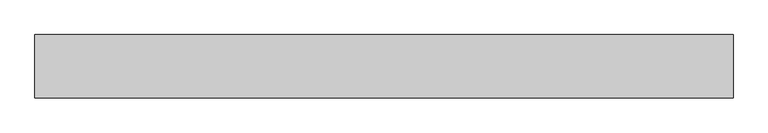
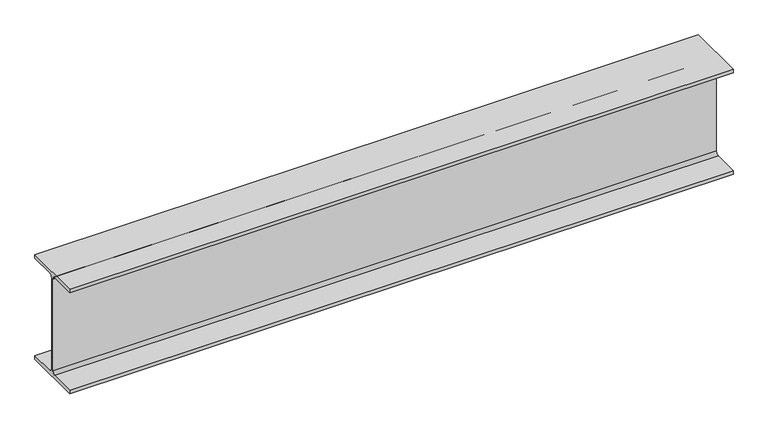
"""IFC4 building model written with IfcOpenShell, lengths in millimetres: beam geometry, Old_Steel Beam_H-KSD3502 : H_SB_ASB_H-200×200x8x12."""

import ifcopenshell
import ifcopenshell.guid

model = None  # the IFC model being written
_history = None  # IfcOwnerHistory: only IFC2X3 demands one
_inside = {}  # id of a spatial element -> (the spatial element, [elements in it])
_under = {}  # id of a project, library or spatial element -> (it, [spatial elements below it])
_declared = {}  # id of a project -> (the project, [libraries it declares])
_typed = {}  # id of a type object -> (the type object, [elements of that type])
_made_of = {}  # id of a material, layer set ... -> (it, [elements and type objects made of it])


def new_model(schema):
    """Start an empty IFC model of exactly this schema.

    Asked for "IFC4X3", IfcOpenShell would pick the latest addendum, in which some entities
    have other attributes; the version numbers below select the first issue.
    IFC2X3 requires an IfcOwnerHistory on every rooted entity: one is made here for all.
    """
    global model, _history
    if schema == "IFC4X3":
        model = ifcopenshell.file(schema_version=(4, 3, 0, 0))
    else:
        model = ifcopenshell.file(schema=schema)
    _inside.clear()
    _under.clear()
    _declared.clear()
    _typed.clear()
    _made_of.clear()
    _history = None
    if model.schema == "IFC2X3":
        org = make("IfcOrganization", Name="unknown")
        user = make(
            "IfcPersonAndOrganization",
            ThePerson=make("IfcPerson", FamilyName="unknown"),
            TheOrganization=org,
        )
        app = make(
            "IfcApplication",
            ApplicationDeveloper=org,
            Version="unknown",
            ApplicationFullName="unknown",
            ApplicationIdentifier="unknown",
        )
        _history = make(
            "IfcOwnerHistory",
            OwningUser=user,
            OwningApplication=app,
            ChangeAction="ADDED",
            CreationDate=0,
        )
    return model


def make(cls, **values):
    """One entity of the class cls with the attributes given. An attribute that is None is left unset."""
    return model.create_entity(
        cls, **{name: value for name, value in values.items() if value is not None}
    )


def rooted(cls, **values):
    """An entity with a GlobalId (a new one), such as an element, a storey or a relation."""
    return make(cls, GlobalId=ifcopenshell.guid.new(), OwnerHistory=_history, **values)


def si_unit(unit_type, name, prefix=None):
    """IfcSIUnit, for example si_unit("LENGTHUNIT", "METRE", prefix="MILLI")."""
    return make("IfcSIUnit", UnitType=unit_type, Prefix=prefix, Name=name)


def assignment(units):
    """IfcUnitAssignment: the units of a project."""
    return None if units is None else make("IfcUnitAssignment", Units=units)


def point(xyz):
    """IfcCartesianPoint."""
    return None if xyz is None else make("IfcCartesianPoint", Coordinates=xyz)


def direction(xyz):
    """IfcDirection."""
    return None if xyz is None else make("IfcDirection", DirectionRatios=xyz)


def frame(location, z_axis=None, x_axis=None):
    """IfcAxis2Placement3D, a coordinate frame: its origin and axes. An axis left out is left unset."""
    return make(
        "IfcAxis2Placement3D",
        Location=point(location),
        Axis=direction(z_axis),
        RefDirection=direction(x_axis),
    )


def frame_2d(location, x_axis=None):
    """IfcAxis2Placement2D, a coordinate frame in the plane: its origin and x axis."""
    return make(
        "IfcAxis2Placement2D", Location=point(location), RefDirection=direction(x_axis)
    )


def origin():
    """The frame at (0, 0, 0) with its axes left unset."""
    return frame((0.0, 0.0, 0.0))


def place(relative_to, where):
    """IfcLocalPlacement: puts the frame where relative to a parent placement (None: the world)."""
    return make(
        "IfcLocalPlacement", PlacementRelTo=relative_to, RelativePlacement=where
    )


def context(
    kind, dimensions, precision=None, world=None, true_north=None, identifier=None
):
    """IfcGeometricRepresentationContext, for example the 3D "Model" context."""
    return make(
        "IfcGeometricRepresentationContext",
        ContextIdentifier=identifier,
        ContextType=kind,
        CoordinateSpaceDimension=dimensions,
        Precision=precision,
        WorldCoordinateSystem=world,
        TrueNorth=true_north,
    )


def project(units=None, contexts=None):
    """IfcProject with its units and contexts."""
    return rooted(
        "IfcProject",
        Name="project",
        RepresentationContexts=contexts,
        UnitsInContext=assignment(units),
    )


def spatial(cls, under=None, at=None, **own):
    """A site, building, storey or space (cls), placed at a placement, below another one or the project."""
    s = rooted(cls, ObjectPlacement=at, **own)
    if under is not None:
        _under.setdefault(under.id(), (under, []))[1].append(s)
    return s


def polyline(points):
    """IfcPolyline through the points."""
    return make("IfcPolyline", Points=[point(p) for p in points])


def circle_curve(where, radius):
    """IfcCircle in the frame where."""
    return make("IfcCircle", Position=where, Radius=radius)


def trimmed(basis, trim1, trim2, sense, master):
    """IfcTrimmedCurve: the piece of a basis curve between two trims."""
    return make(
        "IfcTrimmedCurve",
        BasisCurve=basis,
        Trim1=trim1,
        Trim2=trim2,
        SenseAgreement=sense,
        MasterRepresentation=master,
    )


def segment(curve, same_sense, transition):
    """IfcCompositeCurveSegment."""
    return make(
        "IfcCompositeCurveSegment",
        Transition=transition,
        SameSense=same_sense,
        ParentCurve=curve,
    )


def composite_curve(segments, self_intersect=None):
    """IfcCompositeCurve: segments joined end to end."""
    return make("IfcCompositeCurve", Segments=segments, SelfIntersect=self_intersect)


def outline(outer, holes=None, kind="AREA"):
    """IfcArbitraryClosedProfileDef: a profile drawn as a closed curve; with holes, ...WithVoids."""
    if holes is None:
        return make("IfcArbitraryClosedProfileDef", ProfileType=kind, OuterCurve=outer)
    return make(
        "IfcArbitraryProfileDefWithVoids",
        ProfileType=kind,
        OuterCurve=outer,
        InnerCurves=holes,
    )


def extrude(swept, where, along, depth):
    """IfcExtrudedAreaSolid: the profile swept, set in the frame where, extruded along a direction by depth."""
    return make(
        "IfcExtrudedAreaSolid",
        SweptArea=swept,
        Position=where,
        ExtrudedDirection=direction(along),
        Depth=depth,
    )


def shape(context_of_items, identifier, shape_type, items):
    """IfcShapeRepresentation: the items that make up one representation, for example the "Body"."""
    return make(
        "IfcShapeRepresentation",
        ContextOfItems=context_of_items,
        RepresentationIdentifier=identifier,
        RepresentationType=shape_type,
        Items=items,
    )


def source(mapping_origin, context_of_items, identifier, shape_type, items):
    """IfcRepresentationMap: a shape defined once, which mapped items show again and again."""
    return make(
        "IfcRepresentationMap",
        MappingOrigin=mapping_origin,
        MappedRepresentation=shape(context_of_items, identifier, shape_type, items),
    )


def transform(
    local_origin,
    x_axis=None,
    y_axis=None,
    z_axis=None,
    scale=None,
    scale2=None,
    scale3=None,
    uniform=True,
):
    """IfcCartesianTransformationOperator3D, or its non-uniform kind. x_axis, y_axis, z_axis: its Axis1, 2, 3."""
    if uniform:
        return make(
            "IfcCartesianTransformationOperator3D",
            Axis1=direction(x_axis),
            Axis2=direction(y_axis),
            LocalOrigin=point(local_origin),
            Scale=scale,
            Axis3=direction(z_axis),
        )
    return make(
        "IfcCartesianTransformationOperator3DnonUniform",
        Axis1=direction(x_axis),
        Axis2=direction(y_axis),
        LocalOrigin=point(local_origin),
        Scale=scale,
        Axis3=direction(z_axis),
        Scale2=scale2,
        Scale3=scale3,
    )


def mapped(mapping_source, mapping_target):
    """IfcMappedItem: shows the shape of a source again, moved by a transform."""
    return make(
        "IfcMappedItem", MappingSource=mapping_source, MappingTarget=mapping_target
    )


def made_of(thing, what):
    """Note that an element or type object is made of a material, layer set ...; save() writes the relation."""
    if what is not None:
        _made_of.setdefault(what.id(), (what, []))[1].append(thing)
    return thing


def element(
    cls,
    number,
    at=None,
    inside=None,
    cuts=None,
    type_object=None,
    material=None,
    context=None,
    identifier="Body",
    shape_type=None,
    held_by="IfcProductDefinitionShape",
    body=None,
    shapes=None,
    **own,
):
    """One element of the class cls, such as IfcWall. Its Tag is "e" and its number.

    at: its placement. inside: the storey or other place that contains it. cuts: it is an
    opening in that element (IfcRelVoidsElement). A single representation is given by context,
    identifier, shape_type and body (its items); several are given by shapes. held_by: the class
    of the entity that holds the representations. save() writes the other relations.
    """
    e = rooted(cls, Tag="e%d" % number, ObjectPlacement=at, **own)
    if body is not None:
        shapes = [shape(context, identifier, shape_type, body)]
    if shapes is not None:
        e.Representation = make(held_by, Representations=shapes)
    if inside is not None:
        _inside.setdefault(inside.id(), (inside, []))[1].append(e)
    if cuts is not None:
        rooted(
            "IfcRelVoidsElement", RelatingBuildingElement=cuts, RelatedOpeningElement=e
        )
    if type_object is not None:
        _typed.setdefault(type_object.id(), (type_object, []))[1].append(e)
    return made_of(e, material)


def aggregate(whole, parts):
    """IfcRelAggregates: a whole, such as a stair, and the parts it consists of."""
    return rooted("IfcRelAggregates", RelatingObject=whole, RelatedObjects=parts)


def save(model, path):
    """Write the relations noted so far, then the file.

    IfcRelAggregates (storeys below a building ...), IfcRelContainedInSpatialStructure (elements
    in a storey), IfcRelDefinesByType, IfcRelAssociatesMaterial and IfcRelDeclares: one each for
    every whole, place, type object, material and project.
    """
    for whole, parts in _under.values():
        aggregate(whole, parts)
    for where, things in _inside.values():
        rooted(
            "IfcRelContainedInSpatialStructure",
            RelatedElements=things,
            RelatingStructure=where,
        )
    for kind, things in _typed.values():
        rooted("IfcRelDefinesByType", RelatedObjects=things, RelatingType=kind)
    for what, things in _made_of.values():
        rooted("IfcRelAssociatesMaterial", RelatedObjects=things, RelatingMaterial=what)
    for by, libraries in _declared.values():
        rooted("IfcRelDeclares", RelatingContext=by, RelatedDefinitions=libraries)
    model.write(path)


def beam_2b48dec8(model_context):
    return source(origin(), model_context, "Body", "SweptSolid", [
        extrude(outline(composite_curve([segment(polyline([(82.5, -141.5), (82.5, -151.7), (-82.5, -151.7), (-82.5, -141.5), (-11.9, -141.5)]), True, "CONTINUOUS"), segment(trimmed(circle_curve(frame_2d((-11.9, -132.6)), 8.9), [point((-11.9, -141.5))], [point((-3.0, -132.6))], True, "CARTESIAN"), True, "CONTINUOUS"), segment(polyline([(-3.0, -132.6), (-3.0, 132.6)]), True, "CONTINUOUS"), segment(trimmed(circle_curve(frame_2d((-11.9, 132.6)), 8.9), [point((-3.0, 132.6))], [point((-11.9, 141.5))], True, "CARTESIAN"), True, "CONTINUOUS"), segment(polyline([(-11.9, 141.5), (-82.5, 141.5), (-82.5, 151.7), (82.5, 151.7), (82.5, 141.5), (11.9, 141.5)]), True, "CONTINUOUS"), segment(trimmed(circle_curve(frame_2d((11.9, 132.6)), 8.9), [point((11.9, 141.5))], [point((3.0, 132.6))], True, "CARTESIAN"), True, "CONTINUOUS"), segment(polyline([(3.0, 132.6), (3.0, -132.6)]), True, "CONTINUOUS"), segment(trimmed(circle_curve(frame_2d((11.9, -132.6)), 8.9), [point((3.0, -132.6))], [point((11.9, -141.5))], True, "CARTESIAN"), True, "CONTINUOUS"), segment(polyline([(11.9, -141.5), (82.5, -141.5)]), True, "CONTINUOUS")], self_intersect=False)), frame((-1035.0333333, 0.0, 0.0), z_axis=(1.0, 0.0, 0.0), x_axis=(0.0, 1.0, 0.0)), (0.0, 0.0, 1.0), 1820.0666667),
    ])


if __name__ == "__main__":
    model = new_model("IFC4")
    model_context = context("Model", 3, world=origin())
    ifc_project = project(units=[si_unit("LENGTHUNIT", "METRE", prefix="MILLI")], contexts=[model_context])
    site = spatial("IfcSite", under=ifc_project)
    building = spatial("IfcBuilding", under=site)
    placement = place(None, origin())
    beam_shape = beam_2b48dec8(model_context)
    element("IfcBeam", 1, ObjectType="Old_Steel Beam_H-KSD3502 : H_SB_ASB_H-200×200x8x12", at=placement, inside=building, context=model_context, shape_type="MappedRepresentation", body=[
        mapped(beam_shape, transform((0.0, 0.0, 0.0), x_axis=(1.0, 0.0, 0.0), y_axis=(0.0, 1.0, 0.0), z_axis=(0.0, 0.0, 1.0))),
    ])
    save(model, "model.ifc")

# Revit data of these elements
# Type "Old_Steel Beam_H-KSD3502 : H_SB_ASB_H-200×200x8x12"
#   Width = 20.0 cm
#   Web Thickness = 0.8 cm
#   Web Fillet = 1.3 cm
#   Warping Constant = 141376.0 cm⁶
#   Torsional Moment of Inertia = 26.2485 cm⁴
#   Torsional Modulus = 1.0 cm³
#   Section Area = 63.53 cm²
#   Plastic Modulus weak axis = 244.0 cm³
#   Plastic Modulus strong axis = 525.0 cm³
#   Perimeter = 1.16 m²/m
#   Nominal Weight = 49.90 kgf/m
#   Moment of Inertia weak axis = 1600.00 cm⁴
#   Moment of Inertia strong axis = 4720.00 cm⁴
#   Height = 20.0 cm
#   Flange Thickness = 1.2 cm
#   Elastic Modulus weak axis = 160.0 cm³
#   Elastic Modulus strong axis = 472.0 cm³
#   Centroid Vertical = 10.0 cm
#   Centroid Horizontal = 10.0 cm
#   Length [instance default] = 1.5240 m
#   Structural Material [instance default] = Steel, 45-345
#   Assembly Code = ""
# Element 1 (IfcBeam, "Old_Steel Beam_H-KSD3502 : H_SB_ASB_H-200×200x8x12")
#   Structural Material = none
# Materials
#   "Steel, 45-345": class "Metal", colour RGB 189 187 185, transparency 0, Description = "Steel 345 MPa", Cost = 0
